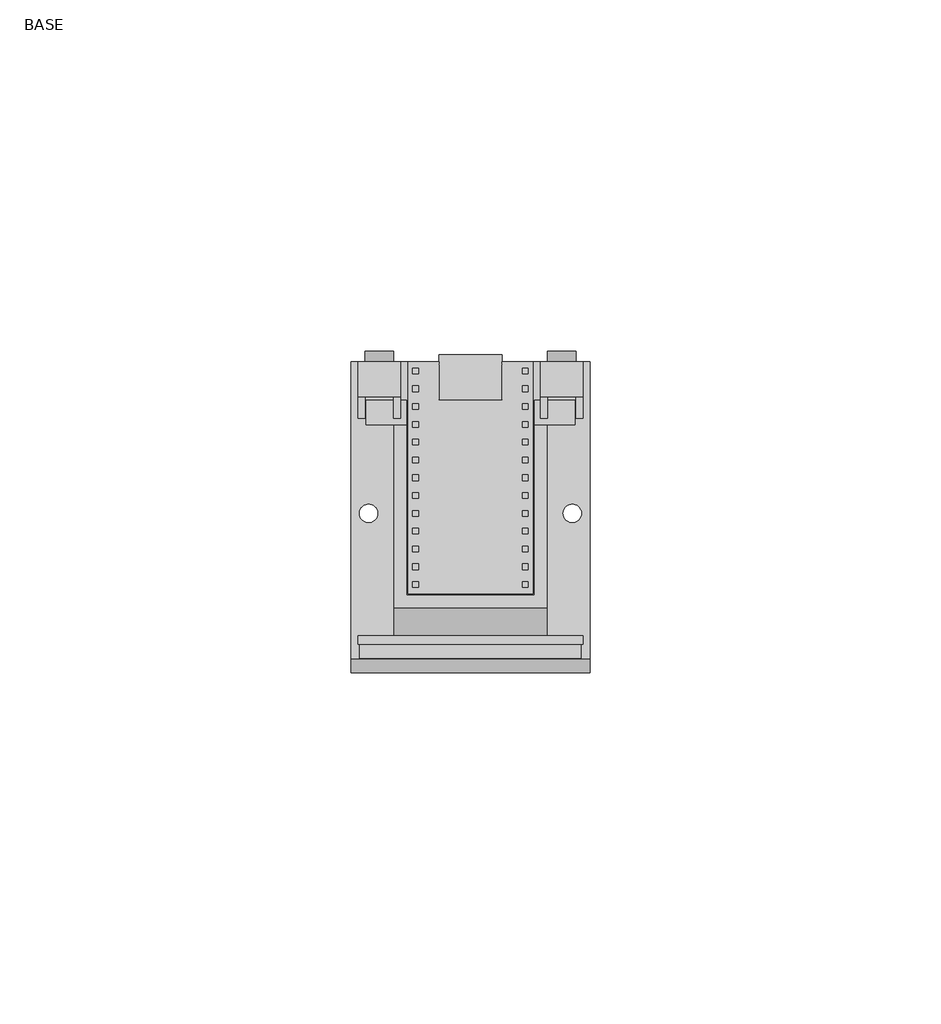
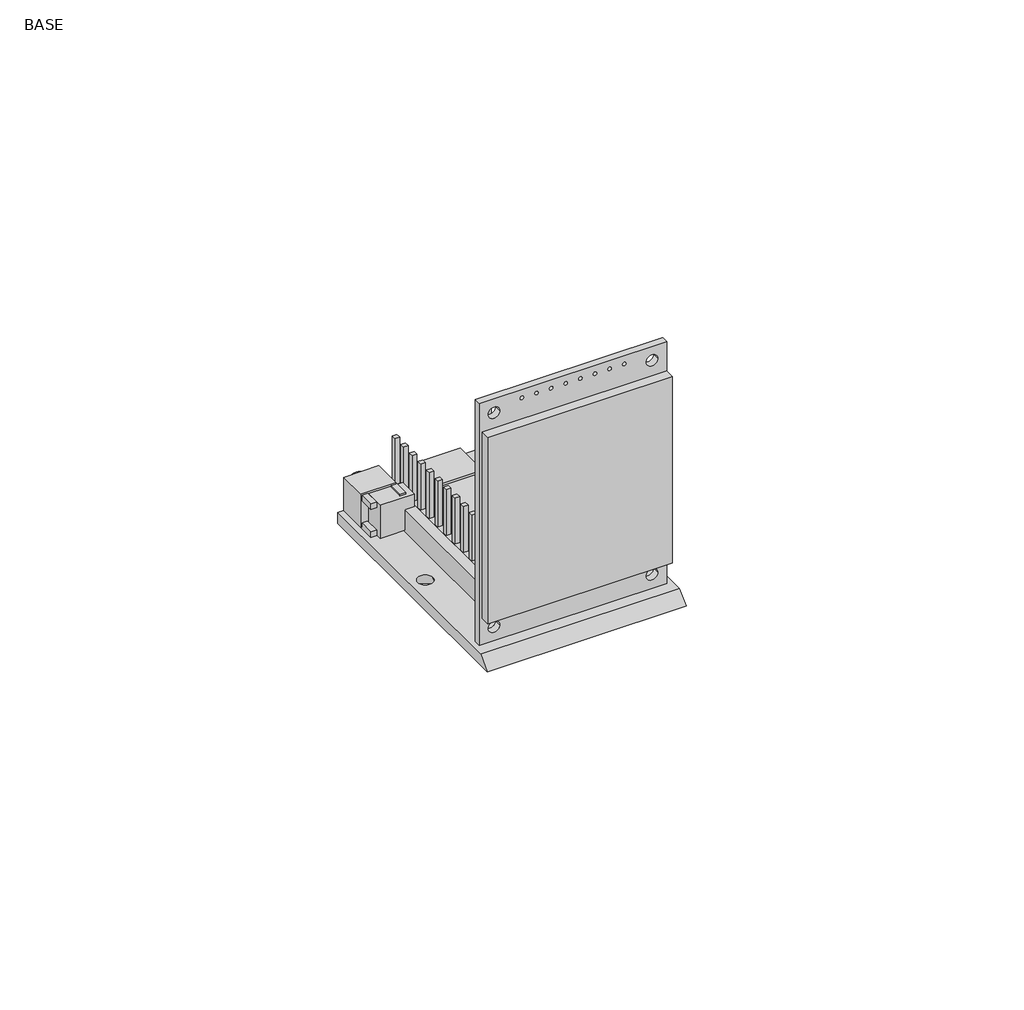
# One storey: 4 furniture elements, 1 proxy.
"""IFC4 building model written with IfcOpenShell, lengths in millimetres."""

import ifcopenshell
import ifcopenshell.guid

model = None  # the IFC model being written
_history = None  # IfcOwnerHistory: only IFC2X3 demands one
_inside = {}  # id of a spatial element -> (the spatial element, [elements in it])
_under = {}  # id of a project, library or spatial element -> (it, [spatial elements below it])
_declared = {}  # id of a project -> (the project, [libraries it declares])
_typed = {}  # id of a type object -> (the type object, [elements of that type])
_made_of = {}  # id of a material, layer set ... -> (it, [elements and type objects made of it])


def new_model(schema):
    """Start an empty IFC model of exactly this schema.

    Asked for "IFC4X3", IfcOpenShell would pick the latest addendum, in which some entities
    have other attributes; the version numbers below select the first issue.
    IFC2X3 requires an IfcOwnerHistory on every rooted entity: one is made here for all.
    """
    global model, _history
    if schema == "IFC4X3":
        model = ifcopenshell.file(schema_version=(4, 3, 0, 0))
    else:
        model = ifcopenshell.file(schema=schema)
    _inside.clear()
    _under.clear()
    _declared.clear()
    _typed.clear()
    _made_of.clear()
    _history = None
    if model.schema == "IFC2X3":
        org = make("IfcOrganization", Name="unknown")
        user = make(
            "IfcPersonAndOrganization",
            ThePerson=make("IfcPerson", FamilyName="unknown"),
            TheOrganization=org,
        )
        app = make(
            "IfcApplication",
            ApplicationDeveloper=org,
            Version="unknown",
            ApplicationFullName="unknown",
            ApplicationIdentifier="unknown",
        )
        _history = make(
            "IfcOwnerHistory",
            OwningUser=user,
            OwningApplication=app,
            ChangeAction="ADDED",
            CreationDate=0,
        )
    return model


def make(cls, **values):
    """One entity of the class cls with the attributes given. An attribute that is None is left unset."""
    return model.create_entity(
        cls, **{name: value for name, value in values.items() if value is not None}
    )


def rooted(cls, **values):
    """An entity with a GlobalId (a new one), such as an element, a storey or a relation."""
    return make(cls, GlobalId=ifcopenshell.guid.new(), OwnerHistory=_history, **values)


def si_unit(unit_type, name, prefix=None):
    """IfcSIUnit, for example si_unit("LENGTHUNIT", "METRE", prefix="MILLI")."""
    return make("IfcSIUnit", UnitType=unit_type, Prefix=prefix, Name=name)


def assignment(units):
    """IfcUnitAssignment: the units of a project."""
    return None if units is None else make("IfcUnitAssignment", Units=units)


def point(xyz):
    """IfcCartesianPoint."""
    return None if xyz is None else make("IfcCartesianPoint", Coordinates=xyz)


def direction(xyz):
    """IfcDirection."""
    return None if xyz is None else make("IfcDirection", DirectionRatios=xyz)


def frame(location, z_axis=None, x_axis=None):
    """IfcAxis2Placement3D, a coordinate frame: its origin and axes. An axis left out is left unset."""
    return make(
        "IfcAxis2Placement3D",
        Location=point(location),
        Axis=direction(z_axis),
        RefDirection=direction(x_axis),
    )


def frame_2d(location, x_axis=None):
    """IfcAxis2Placement2D, a coordinate frame in the plane: its origin and x axis."""
    return make(
        "IfcAxis2Placement2D", Location=point(location), RefDirection=direction(x_axis)
    )


def origin():
    """The frame at (0, 0, 0) with its axes left unset."""
    return frame((0.0, 0.0, 0.0))


def origin_with_axes():
    """The frame at (0, 0, 0) with the z axis (0, 0, 1) and the x axis (1, 0, 0) written out."""
    return frame((0.0, 0.0, 0.0), z_axis=(0.0, 0.0, 1.0), x_axis=(1.0, 0.0, 0.0))


def place(relative_to, where):
    """IfcLocalPlacement: puts the frame where relative to a parent placement (None: the world)."""
    return make(
        "IfcLocalPlacement", PlacementRelTo=relative_to, RelativePlacement=where
    )


def context(
    kind, dimensions, precision=None, world=None, true_north=None, identifier=None
):
    """IfcGeometricRepresentationContext, for example the 3D "Model" context."""
    return make(
        "IfcGeometricRepresentationContext",
        ContextIdentifier=identifier,
        ContextType=kind,
        CoordinateSpaceDimension=dimensions,
        Precision=precision,
        WorldCoordinateSystem=world,
        TrueNorth=true_north,
    )


def project(units=None, contexts=None):
    """IfcProject with its units and contexts."""
    return rooted(
        "IfcProject",
        Name="project",
        RepresentationContexts=contexts,
        UnitsInContext=assignment(units),
    )


def spatial(cls, under=None, at=None, **own):
    """A site, building, storey or space (cls), placed at a placement, below another one or the project."""
    s = rooted(cls, ObjectPlacement=at, **own)
    if under is not None:
        _under.setdefault(under.id(), (under, []))[1].append(s)
    return s


def polyline(points):
    """IfcPolyline through the points."""
    return make("IfcPolyline", Points=[point(p) for p in points])


def circle_curve(where, radius):
    """IfcCircle in the frame where."""
    return make("IfcCircle", Position=where, Radius=radius)


def trimmed(basis, trim1, trim2, sense, master):
    """IfcTrimmedCurve: the piece of a basis curve between two trims."""
    return make(
        "IfcTrimmedCurve",
        BasisCurve=basis,
        Trim1=trim1,
        Trim2=trim2,
        SenseAgreement=sense,
        MasterRepresentation=master,
    )


def segment(curve, same_sense, transition):
    """IfcCompositeCurveSegment."""
    return make(
        "IfcCompositeCurveSegment",
        Transition=transition,
        SameSense=same_sense,
        ParentCurve=curve,
    )


def composite_curve(segments, self_intersect=None):
    """IfcCompositeCurve: segments joined end to end."""
    return make("IfcCompositeCurve", Segments=segments, SelfIntersect=self_intersect)


def outline(outer, holes=None, kind="AREA"):
    """IfcArbitraryClosedProfileDef: a profile drawn as a closed curve; with holes, ...WithVoids."""
    if holes is None:
        return make("IfcArbitraryClosedProfileDef", ProfileType=kind, OuterCurve=outer)
    return make(
        "IfcArbitraryProfileDefWithVoids",
        ProfileType=kind,
        OuterCurve=outer,
        InnerCurves=holes,
    )


def extrude(swept, where, along, depth):
    """IfcExtrudedAreaSolid: the profile swept, set in the frame where, extruded along a direction by depth."""
    return make(
        "IfcExtrudedAreaSolid",
        SweptArea=swept,
        Position=where,
        ExtrudedDirection=direction(along),
        Depth=depth,
    )


def faces_of(points, faces, orient=None, outer=None):
    """IfcFace entities. A face is a list of loops; a loop is a list of indices into points, from 0.

    orient and outer hold one flag for each loop. By default every Orientation is true, the
    first loop of a face is its IfcFaceOuterBound and the others are IfcFaceBound.
    """
    made = []
    for i, loops in enumerate(faces):
        bounds = []
        for j, loop in enumerate(loops):
            is_outer = j == 0 if outer is None else outer[i][j]
            bounds.append(
                make(
                    "IfcFaceOuterBound" if is_outer else "IfcFaceBound",
                    Bound=make("IfcPolyLoop", Polygon=[points[k] for k in loop]),
                    Orientation=True if orient is None else orient[i][j],
                )
            )
        made.append(make("IfcFace", Bounds=bounds))
    return made


def faceted_brep(points, faces, orient=None, outer=None, voids=None):
    """IfcFacetedBrep: a solid bounded by flat faces; with voids (closed shells), ...WithVoids."""
    shared = [point(p) for p in points]
    hull = make("IfcClosedShell", CfsFaces=faces_of(shared, faces, orient, outer))
    if voids is None:
        return make("IfcFacetedBrep", Outer=hull)
    return make(
        "IfcFacetedBrepWithVoids",
        Outer=hull,
        Voids=[
            make(cls, CfsFaces=faces_of(shared, fs, o, b)) for cls, fs, o, b in voids
        ],
    )


def shape(context_of_items, identifier, shape_type, items):
    """IfcShapeRepresentation: the items that make up one representation, for example the "Body"."""
    return make(
        "IfcShapeRepresentation",
        ContextOfItems=context_of_items,
        RepresentationIdentifier=identifier,
        RepresentationType=shape_type,
        Items=items,
    )


def source(mapping_origin, context_of_items, identifier, shape_type, items):
    """IfcRepresentationMap: a shape defined once, which mapped items show again and again."""
    return make(
        "IfcRepresentationMap",
        MappingOrigin=mapping_origin,
        MappedRepresentation=shape(context_of_items, identifier, shape_type, items),
    )


def transform(
    local_origin,
    x_axis=None,
    y_axis=None,
    z_axis=None,
    scale=None,
    scale2=None,
    scale3=None,
    uniform=True,
):
    """IfcCartesianTransformationOperator3D, or its non-uniform kind. x_axis, y_axis, z_axis: its Axis1, 2, 3."""
    if uniform:
        return make(
            "IfcCartesianTransformationOperator3D",
            Axis1=direction(x_axis),
            Axis2=direction(y_axis),
            LocalOrigin=point(local_origin),
            Scale=scale,
            Axis3=direction(z_axis),
        )
    return make(
        "IfcCartesianTransformationOperator3DnonUniform",
        Axis1=direction(x_axis),
        Axis2=direction(y_axis),
        LocalOrigin=point(local_origin),
        Scale=scale,
        Axis3=direction(z_axis),
        Scale2=scale2,
        Scale3=scale3,
    )


def mapped(mapping_source, mapping_target):
    """IfcMappedItem: shows the shape of a source again, moved by a transform."""
    return make(
        "IfcMappedItem", MappingSource=mapping_source, MappingTarget=mapping_target
    )


def made_of(thing, what):
    """Note that an element or type object is made of a material, layer set ...; save() writes the relation."""
    if what is not None:
        _made_of.setdefault(what.id(), (what, []))[1].append(thing)
    return thing


def element(
    cls,
    number,
    at=None,
    inside=None,
    cuts=None,
    type_object=None,
    material=None,
    context=None,
    identifier="Body",
    shape_type=None,
    held_by="IfcProductDefinitionShape",
    body=None,
    shapes=None,
    **own,
):
    """One element of the class cls, such as IfcWall. Its Tag is "e" and its number.

    at: its placement. inside: the storey or other place that contains it. cuts: it is an
    opening in that element (IfcRelVoidsElement). A single representation is given by context,
    identifier, shape_type and body (its items); several are given by shapes. held_by: the class
    of the entity that holds the representations. save() writes the other relations.
    """
    e = rooted(cls, Tag="e%d" % number, ObjectPlacement=at, **own)
    if body is not None:
        shapes = [shape(context, identifier, shape_type, body)]
    if shapes is not None:
        e.Representation = make(held_by, Representations=shapes)
    if inside is not None:
        _inside.setdefault(inside.id(), (inside, []))[1].append(e)
    if cuts is not None:
        rooted(
            "IfcRelVoidsElement", RelatingBuildingElement=cuts, RelatedOpeningElement=e
        )
    if type_object is not None:
        _typed.setdefault(type_object.id(), (type_object, []))[1].append(e)
    return made_of(e, material)


def aggregate(whole, parts):
    """IfcRelAggregates: a whole, such as a stair, and the parts it consists of."""
    return rooted("IfcRelAggregates", RelatingObject=whole, RelatedObjects=parts)


def save(model, path):
    """Write the relations noted so far, then the file.

    IfcRelAggregates (storeys below a building ...), IfcRelContainedInSpatialStructure (elements
    in a storey), IfcRelDefinesByType, IfcRelAssociatesMaterial and IfcRelDeclares: one each for
    every whole, place, type object, material and project.
    """
    for whole, parts in _under.values():
        aggregate(whole, parts)
    for where, things in _inside.values():
        rooted(
            "IfcRelContainedInSpatialStructure",
            RelatedElements=things,
            RelatingStructure=where,
        )
    for kind, things in _typed.values():
        rooted("IfcRelDefinesByType", RelatedObjects=things, RelatingType=kind)
    for what, things in _made_of.values():
        rooted("IfcRelAssociatesMaterial", RelatedObjects=things, RelatingMaterial=what)
    for by, libraries in _declared.values():
        rooted("IfcRelDeclares", RelatingContext=by, RelatedDefinitions=libraries)
    model.write(path)


def plane_surface(at):
    """IfcPlane: the flat surface through the origin of the frame at, square to its z axis."""
    return make("IfcPlane", Position=at)


def revolved_surface(curve, axis_point, axis_direction):
    """IfcSurfaceOfRevolution: the curve turned about the line through axis_point along axis_direction."""
    return make(
        "IfcSurfaceOfRevolution",
        SweptCurve=make("IfcArbitraryOpenProfileDef", ProfileType="CURVE", Curve=curve),
        AxisPosition=make("IfcAxis1Placement", Location=point(axis_point), Axis=direction(axis_direction)),
    )


def advanced_brep(points, edges, surfaces, faces):
    """IfcAdvancedBrep: a solid bounded by faces that lie on surfaces and meet in shared edges.

    An edge is (start, end): straight between two places in points (the first is 0);
    or (start, end, curve); or (start, end, curve, False) where it runs against its curve.
    A face is (place in surfaces, loops), or (place, loops, False) where it looks against
    its surface's normal. A loop lists edges by number (the first is 1), with a minus sign
    where the edge is run from its end to its start. The first loop is the outer one.
    """
    corners = [point(p) for p in points]
    vertices = [make("IfcVertexPoint", VertexGeometry=c) for c in corners]
    made = []
    for start, end, *more in edges:
        made.append(
            make(
                "IfcEdgeCurve",
                EdgeStart=vertices[start],
                EdgeEnd=vertices[end],
                EdgeGeometry=more[0] if more else make("IfcPolyline", Points=[corners[start], corners[end]]),
                SameSense=more[1] if len(more) > 1 else True,
            )
        )
    hull = []
    for where, loops, *sense in faces:
        bounds = []
        for j, loop in enumerate(loops):
            ring = [make("IfcOrientedEdge", EdgeElement=made[abs(k) - 1], Orientation=k > 0) for k in loop]
            bounds.append(
                make(
                    "IfcFaceOuterBound" if j == 0 else "IfcFaceBound",
                    Bound=make("IfcEdgeLoop", EdgeList=ring),
                    Orientation=True,
                )
            )
        hull.append(make("IfcAdvancedFace", Bounds=bounds, FaceSurface=surfaces[where], SameSense=sense[0] if sense else True))
    return make("IfcAdvancedBrep", Outer=make("IfcClosedShell", CfsFaces=hull))


def case_case_ec59ddf9(model_context):
    return source(origin(), model_context, "Body", "SolidModel", [
        extrude(outline(polyline([(1461.1150176, 13229.1739696), (1466.9150176, 13229.1739696), (1466.9150176, 13225.7186096), (1461.1150176, 13225.7186096), (1461.1150176, 13229.1739696)])), frame((0.0, 0.0, 2.0), z_axis=(0.0, 0.0, 1.0), x_axis=(1.0, 0.0, 0.0)), (0.0, 0.0, 1.0), 6.0),
        extrude(outline(polyline([(1442.9350176, 13229.1739696), (1442.9350176, 13225.7186096), (1437.1350176, 13225.7186096), (1437.1350176, 13229.1739696), (1442.9350176, 13229.1739696)])), frame((0.0, 0.0, 2.0), z_axis=(0.0, 0.0, 1.0), x_axis=(1.0, 0.0, 0.0)), (0.0, 0.0, 1.0), 6.0),
        advanced_brep(
        [(1469.0250176, 13192.4212784, 2.0), (1469.0250176, 13234.6739696, 2.0), (1435.0250176, 13234.6739696, 2.0), (1435.0250176, 13192.4212784, 2.0), (1441.1350176, 13195.6739696, 2.0), (1441.1350176, 13225.7186096, 2.0), (1442.9350176, 13225.7186096, 2.0), (1442.9350176, 13201.4739696, 2.0), (1461.1150176, 13201.4739696, 2.0), (1461.1150176, 13225.7186096, 2.0), (1462.9150176, 13225.7186096, 2.0), (1462.9150176, 13195.6739696, 2.0), (1467.8250176, 13213.1041412, 2.0), (1465.2250176, 13213.1041412, 2.0), (1438.8250176, 13213.1041412, 2.0), (1436.2250176, 13213.1041412, 2.0), (1435.0250176, 13234.6739696, 0.0), (1469.0250176, 13234.6739696, 0.0), (1469.0250176, 13190.4212784, 0.0), (1435.0250176, 13190.4212784, 0.0), (1464.5250176, 13213.1041412, 0.0), (1468.5250176, 13213.1041412, 0.0), (1435.5250176, 13213.1041412, 0.0), (1439.5250176, 13213.1041412, 0.0), (1441.1350176, 13225.7186096, 6.0), (1441.1350176, 13199.6739696, 6.0), (1462.9150176, 13199.6739696, 6.0), (1462.9150176, 13225.7186096, 6.0), (1461.1150176, 13225.7186096, 6.0), (1461.1150176, 13201.4739696, 6.0), (1442.9350176, 13201.4739696, 6.0), (1442.9350176, 13225.7186096, 6.0)],
        [
            (0, 1),
            (1, 2),
            (2, 3),
            (3, 0),
            (4, 5),
            (5, 6),
            (6, 7),
            (7, 8),
            (8, 9),
            (9, 10),
            (10, 11),
            (11, 4),
            (12, 13, circle_curve(frame((1466.5250176, 13213.1041412, 2.0), z_axis=(0.0, 0.0, -1.0), x_axis=(-1.0, 0.0, 0.0)), 1.3)),
            (13, 12, circle_curve(frame((1466.5250176, 13213.1041412, 2.0), z_axis=(0.0, 0.0, -1.0), x_axis=(1.0, 0.0, 0.0)), 1.3)),
            (14, 15, circle_curve(frame((1437.5250176, 13213.1041412, 2.0), z_axis=(0.0, 0.0, -1.0), x_axis=(-1.0, 0.0, 0.0)), 1.3)),
            (15, 14, circle_curve(frame((1437.5250176, 13213.1041412, 2.0), z_axis=(0.0, 0.0, -1.0), x_axis=(1.0, 0.0, 0.0)), 1.3)),
            (16, 17),
            (17, 18),
            (18, 19),
            (19, 16),
            (20, 21, circle_curve(frame((1466.5250176, 13213.1041412, 0.0), z_axis=(0.0, 0.0, 1.0), x_axis=(-1.0, 0.0, 0.0)), 2.0)),
            (21, 20, circle_curve(frame((1466.5250176, 13213.1041412, 0.0), z_axis=(0.0, 0.0, 1.0), x_axis=(1.0, 0.0, 0.0)), 2.0)),
            (22, 23, circle_curve(frame((1437.5250176, 13213.1041412, 0.0), z_axis=(0.0, 0.0, 1.0), x_axis=(-1.0, 0.0, 0.0)), 2.0)),
            (23, 22, circle_curve(frame((1437.5250176, 13213.1041412, 0.0), z_axis=(0.0, 0.0, 1.0), x_axis=(1.0, 0.0, 0.0)), 2.0)),
            (0, 18),
            (17, 1),
            (16, 2),
            (19, 3),
            (24, 25),
            (25, 26),
            (26, 27),
            (27, 28),
            (28, 29),
            (29, 30),
            (30, 31),
            (31, 24),
            (24, 5),
            (4, 25),
            (26, 11),
            (10, 27),
            (9, 28),
            (8, 29),
            (7, 30),
            (6, 31),
            (20, 13),
            (12, 21),
            (22, 15),
            (14, 23),
        ],
        [
            plane_surface(frame((1467.7850176, 13192.4212784, 2.0), z_axis=(0.0, 0.0, 1.0), x_axis=(1.0, 0.0, 0.0))),
            plane_surface(frame((1467.7850176, 13192.4212784, 0.0), z_axis=(0.0, 0.0, -1.0), x_axis=(-1.0, 0.0, 0.0))),
            plane_surface(frame((1469.0250176, 13192.4212784, 2.0), z_axis=(1.0, 0.0, 0.0), x_axis=(0.0, 0.0, -1.0))),
            plane_surface(frame((1469.0250176, 13234.6739696, 2.0), z_axis=(0.0, 1.0, 0.0), x_axis=(0.0, 0.0, -1.0))),
            plane_surface(frame((1435.0250176, 13234.6739696, 2.0), z_axis=(-1.0, 0.0, 0.0), x_axis=(0.0, 0.0, -1.0))),
            plane_surface(frame((1441.1350176, 13234.6739696, 6.0), z_axis=(0.0, 0.0, 1.0), x_axis=(0.0, -1.0, 0.0))),
            plane_surface(frame((1441.1350176, 13225.7186096, 6.0), z_axis=(-1.0, 0.0, 0.0), x_axis=(0.0, 0.0, -1.0))),
            plane_surface(frame((1462.9150176, 13199.6739696, 6.0), z_axis=(1.0, 0.0, 0.0), x_axis=(0.0, 0.0, -1.0))),
            plane_surface(frame((1462.9150176, 13225.7186096, 6.0), z_axis=(0.0, 1.0, 0.0), x_axis=(0.0, 0.0, -1.0))),
            plane_surface(frame((1461.1150176, 13225.7186096, 6.0), z_axis=(-1.0, 0.0, 0.0), x_axis=(0.0, 0.0, -1.0))),
            plane_surface(frame((1461.1150176, 13201.4739696, 6.0), z_axis=(0.0, 1.0, 0.0), x_axis=(0.0, 0.0, -1.0))),
            plane_surface(frame((1442.9350176, 13201.4739696, 6.0), z_axis=(1.0, 0.0, 0.0), x_axis=(0.0, 0.0, -1.0))),
            plane_surface(frame((1442.9350176, 13225.7186096, 6.0), z_axis=(0.0, 1.0, 0.0), x_axis=(0.0, 0.0, -1.0))),
            plane_surface(frame((1441.1350176, 13195.6739696, 2.0), z_axis=(0.0, -0.7071067811865885, 0.7071067811865066), x_axis=(1.0, 0.0, 0.0))),
            plane_surface(frame((1435.0250176, 13190.4212784, 0.0), z_axis=(0.0, -0.707106781186628, 0.7071067811864672), x_axis=(1.0, 0.0, 0.0))),
            revolved_surface(polyline([(1464.5250176, 13213.1041412, 0.0), (1465.2250176017499, 13213.1041412, 2.0)]), (1466.5250176, 13213.1041412, 5.7142857), (0.0, 0.0, -1.0)),
            revolved_surface(polyline([(1435.5250176, 13213.1041412, 0.0), (1436.2250176017499, 13213.1041412, 2.0)]), (1437.5250176, 13213.1041412, 5.7142857), (0.0, 0.0, -1.0)),
        ],
        [
            (0, [[1, 2, 3, 4], [5, 6, 7, 8, 9, 10, 11, 12], [13, 14], [15, 16]]),
            (1, [[17, 18, 19, 20], [21, 22], [23, 24]]),
            (2, [[-1, 25, -18, 26]]),
            (3, [[-2, -26, -17, 27]]),
            (4, [[-3, -27, -20, 28]]),
            (5, [[29, 30, 31, 32, 33, 34, 35, 36]]),
            (6, [[-29, 37, -5, 38]]),
            (7, [[-31, 39, -11, 40]]),
            (8, [[-32, -40, -10, 41]]),
            (9, [[-33, -41, -9, 42]]),
            (10, [[-34, -42, -8, 43]]),
            (11, [[-35, -43, -7, 44]]),
            (12, [[-36, -44, -6, -37]]),
            (13, [[-38, -12, -39, -30]]),
            (14, [[-28, -19, -25, -4]]),
            (15, [[45, -13, 46, -21]]),
            (15, [[-45, -22, -46, -14]]),
            (16, [[47, -15, 48, -23]]),
            (16, [[-47, -24, -48, -16]]),
        ],
    ),
    ])


def furniture_1_54tft_screen_1_54tft_screen_d9e98271(model_context):
    return source(origin(), model_context, "Body", "SweptSolid", [
        extrude(outline(polyline([(43.7, 16.0), (43.7, -16.0), (0.0, -16.0), (0.0, 16.0), (43.7, 16.0)]), holes=[composite_curve([segment(trimmed(circle_curve(frame_2d((2.5, 13.5)), 1.0), [point((2.5, 14.5))], [point((2.5, 12.5))], True, "CARTESIAN"), True, "CONTINUOUS"), segment(trimmed(circle_curve(frame_2d((2.5, 13.5)), 1.0), [point((2.5, 12.5))], [point((2.5, 14.5))], True, "CARTESIAN"), True, "CONTINUOUS")], self_intersect=False), composite_curve([segment(trimmed(circle_curve(frame_2d((41.2, 13.5)), 1.0), [point((41.2, 14.5))], [point((41.2, 12.5))], True, "CARTESIAN"), True, "CONTINUOUS"), segment(trimmed(circle_curve(frame_2d((41.2, 13.5)), 1.0), [point((41.2, 12.5))], [point((41.2, 14.5))], True, "CARTESIAN"), True, "CONTINUOUS")], self_intersect=False), composite_curve([segment(trimmed(circle_curve(frame_2d((42.2, -1.25)), 0.3), [point((42.2, -0.95))], [point((42.2, -1.55))], True, "CARTESIAN"), True, "CONTINUOUS"), segment(trimmed(circle_curve(frame_2d((42.2, -1.25)), 0.3), [point((42.2, -1.55))], [point((42.2, -0.95))], True, "CARTESIAN"), True, "CONTINUOUS")], self_intersect=False), composite_curve([segment(trimmed(circle_curve(frame_2d((42.2, 1.25)), 0.3), [point((42.2, 1.55))], [point((42.2, 0.95))], True, "CARTESIAN"), True, "CONTINUOUS"), segment(trimmed(circle_curve(frame_2d((42.2, 1.25)), 0.3), [point((42.2, 0.95))], [point((42.2, 1.55))], True, "CARTESIAN"), True, "CONTINUOUS")], self_intersect=False), composite_curve([segment(trimmed(circle_curve(frame_2d((42.2, 3.75)), 0.3), [point((42.2, 4.05))], [point((42.2, 3.45))], True, "CARTESIAN"), True, "CONTINUOUS"), segment(trimmed(circle_curve(frame_2d((42.2, 3.75)), 0.3), [point((42.2, 3.45))], [point((42.2, 4.05))], True, "CARTESIAN"), True, "CONTINUOUS")], self_intersect=False), composite_curve([segment(trimmed(circle_curve(frame_2d((42.2, 6.25)), 0.3), [point((42.2, 6.55))], [point((42.2, 5.95))], True, "CARTESIAN"), True, "CONTINUOUS"), segment(trimmed(circle_curve(frame_2d((42.2, 6.25)), 0.3), [point((42.2, 5.95))], [point((42.2, 6.55))], True, "CARTESIAN"), True, "CONTINUOUS")], self_intersect=False), composite_curve([segment(trimmed(circle_curve(frame_2d((42.2, 8.75)), 0.3), [point((42.2, 9.05))], [point((42.2, 8.45))], True, "CARTESIAN"), True, "CONTINUOUS"), segment(trimmed(circle_curve(frame_2d((42.2, 8.75)), 0.3), [point((42.2, 8.45))], [point((42.2, 9.05))], True, "CARTESIAN"), True, "CONTINUOUS")], self_intersect=False), composite_curve([segment(trimmed(circle_curve(frame_2d((42.2, -3.75)), 0.3), [point((42.2, -3.45))], [point((42.2, -4.05))], True, "CARTESIAN"), True, "CONTINUOUS"), segment(trimmed(circle_curve(frame_2d((42.2, -3.75)), 0.3), [point((42.2, -4.05))], [point((42.2, -3.45))], True, "CARTESIAN"), True, "CONTINUOUS")], self_intersect=False), composite_curve([segment(trimmed(circle_curve(frame_2d((42.2, -6.25)), 0.3), [point((42.2, -5.95))], [point((42.2, -6.55))], True, "CARTESIAN"), True, "CONTINUOUS"), segment(trimmed(circle_curve(frame_2d((42.2, -6.25)), 0.3), [point((42.2, -6.55))], [point((42.2, -5.95))], True, "CARTESIAN"), True, "CONTINUOUS")], self_intersect=False), composite_curve([segment(trimmed(circle_curve(frame_2d((42.2, -8.75)), 0.3), [point((42.2, -8.45))], [point((42.2, -9.05))], True, "CARTESIAN"), True, "CONTINUOUS"), segment(trimmed(circle_curve(frame_2d((42.2, -8.75)), 0.3), [point((42.2, -9.05))], [point((42.2, -8.45))], True, "CARTESIAN"), True, "CONTINUOUS")], self_intersect=False), composite_curve([segment(trimmed(circle_curve(frame_2d((41.2, -13.5)), 1.0), [point((41.2, -14.5))], [point((41.2, -12.5))], True, "CARTESIAN"), True, "CONTINUOUS"), segment(trimmed(circle_curve(frame_2d((41.2, -13.5)), 1.0), [point((41.2, -12.5))], [point((41.2, -14.5))], True, "CARTESIAN"), True, "CONTINUOUS")], self_intersect=False), composite_curve([segment(trimmed(circle_curve(frame_2d((2.5, -13.5)), 1.0), [point((2.5, -14.5))], [point((2.5, -12.5))], True, "CARTESIAN"), True, "CONTINUOUS"), segment(trimmed(circle_curve(frame_2d((2.5, -13.5)), 1.0), [point((2.5, -12.5))], [point((2.5, -14.5))], True, "CARTESIAN"), True, "CONTINUOUS")], self_intersect=False)]), frame((0.0, -1.2, 0.0), z_axis=(0.0, 1.0, 0.0), x_axis=(0.0, 0.0, 1.0)), (0.0, 0.0, 1.0), 1.2),
        extrude(outline(polyline([(15.76, -1.3), (15.76, -3.2), (-15.76, -3.2), (-15.76, -1.3), (15.76, -1.3)])), frame((0.0, 0.0, 5.0), z_axis=(0.0, 0.0, 1.0), x_axis=(1.0, 0.0, 0.0)), (0.0, 0.0, 1.0), 33.7),
        extrude(outline(polyline([(13.86, -2.3592442), (13.86, -3.2), (-13.86, -3.2), (-13.86, -2.3592442), (13.86, -2.3592442)])), frame((0.0, 0.0, 9.5994076), z_axis=(0.0, 0.0, 1.0), x_axis=(1.0, 0.0, 0.0)), (0.0, 0.0, 1.0), 27.7),
    ])


def pro_micro_nrf52840_pro_micro_nrf52840_bcfd0b97(model_context):
    return source(origin(), model_context, "Body", "Brep", [
        faceted_brep([(-14.8, 8.2144911, 11.3), (-15.6, 8.2144911, 11.3), (-15.6, 7.4144911, 11.3), (-14.8, 7.4144911, 11.3), (15.6, 8.2144911, 11.3), (14.8, 8.2144911, 11.3), (14.8, 7.4144911, 11.3), (15.6, 7.4144911, 11.3), (13.0666667, 8.2144911, 11.3), (12.2666667, 8.2144911, 11.3), (12.2666667, 7.4144911, 11.3), (13.0666667, 7.4144911, 11.3), (10.5333333, 8.2144911, 11.3), (9.7333333, 8.2144911, 11.3), (9.7333333, 7.4144911, 11.3), (10.5333333, 7.4144911, 11.3), (8.0, 8.2144911, 11.3), (7.2, 8.2144911, 11.3), (7.2, 7.4144911, 11.3), (8.0, 7.4144911, 11.3), (5.4666667, 8.2144911, 11.3), (4.6666667, 8.2144911, 11.3), (4.6666667, 7.4144911, 11.3), (5.4666667, 7.4144911, 11.3), (2.9333333, 8.2144911, 11.3), (2.1333333, 8.2144911, 11.3), (2.1333333, 7.4144911, 11.3), (2.9333333, 7.4144911, 11.3), (0.4, 8.2144911, 11.3), (-0.4, 8.2144911, 11.3), (-0.4, 7.4144911, 11.3), (0.4, 7.4144911, 11.3), (-2.1333333, 8.2144911, 11.3), (-2.9333333, 8.2144911, 11.3), (-2.9333333, 7.4144911, 11.3), (-2.1333333, 7.4144911, 11.3), (-4.6666667, 8.2144911, 11.3), (-5.4666667, 8.2144911, 11.3), (-5.4666667, 7.4144911, 11.3), (-4.6666667, 7.4144911, 11.3), (-7.2, 8.2144911, 11.3), (-8.0, 8.2144911, 11.3), (-8.0, 7.4144911, 11.3), (-7.2, 7.4144911, 11.3), (-9.7333333, 8.2144911, 11.3), (-10.5333333, 8.2144911, 11.3), (-10.5333333, 7.4144911, 11.3), (-9.7333333, 7.4144911, 11.3), (-12.2666667, 8.2144911, 11.3), (-13.0666667, 8.2144911, 11.3), (-13.0666667, 7.4144911, 11.3), (-12.2666667, 7.4144911, 11.3), (-14.8, 8.2144911, 0.0), (-14.8, 7.4144911, 0.0), (-15.6, 7.4144911, 0.0), (-15.6, 8.2144911, 0.0), (15.6, 8.2144911, 0.0), (15.6, 7.4144911, 0.0), (14.8, 7.4144911, 0.0), (14.8, 8.2144911, 0.0), (13.0666667, 8.2144911, 0.0), (13.0666667, 7.4144911, 0.0), (12.2666667, 7.4144911, 0.0), (12.2666667, 8.2144911, 0.0), (10.5333333, 8.2144911, 0.0), (10.5333333, 7.4144911, 0.0), (9.7333333, 7.4144911, 0.0), (9.7333333, 8.2144911, 0.0), (8.0, 8.2144911, 0.0), (8.0, 7.4144911, 0.0), (7.2, 7.4144911, 0.0), (7.2, 8.2144911, 0.0), (5.4666667, 8.2144911, 0.0), (5.4666667, 7.4144911, 0.0), (4.6666667, 7.4144911, 0.0), (4.6666667, 8.2144911, 0.0), (2.9333333, 8.2144911, 0.0), (2.9333333, 7.4144911, 0.0), (2.1333333, 7.4144911, 0.0), (2.1333333, 8.2144911, 0.0), (0.4, 8.2144911, 0.0), (0.4, 7.4144911, 0.0), (-0.4, 7.4144911, 0.0), (-0.4, 8.2144911, 0.0), (-2.1333333, 8.2144911, 0.0), (-2.1333333, 7.4144911, 0.0), (-2.9333333, 7.4144911, 0.0), (-2.9333333, 8.2144911, 0.0), (-4.6666667, 8.2144911, 0.0), (-4.6666667, 7.4144911, 0.0), (-5.4666667, 7.4144911, 0.0), (-5.4666667, 8.2144911, 0.0), (-7.2, 8.2144911, 0.0), (-7.2, 7.4144911, 0.0), (-8.0, 7.4144911, 0.0), (-8.0, 8.2144911, 0.0), (-9.7333333, 8.2144911, 0.0), (-9.7333333, 7.4144911, 0.0), (-10.5333333, 7.4144911, 0.0), (-10.5333333, 8.2144911, 0.0), (-12.2666667, 8.2144911, 0.0), (-12.2666667, 7.4144911, 0.0), (-13.0666667, 7.4144911, 0.0), (-13.0666667, 8.2144911, 0.0), (-14.8, 8.2144911, 3.0), (-15.6, 8.2144911, 3.0), (-15.6, 8.2144911, 1.0), (-14.8, 8.2144911, 1.0), (-15.6, 7.4144911, 3.0), (-15.6, 7.4144911, 1.0), (-14.8, 7.4144911, 3.0), (-14.8, 7.4144911, 1.0), (15.6, 8.2144911, 3.0), (14.8, 8.2144911, 3.0), (14.8, 8.2144911, 1.0), (15.6, 8.2144911, 1.0), (14.8, 7.4144911, 3.0), (14.8, 7.4144911, 1.0), (15.6, 7.4144911, 3.0), (15.6, 7.4144911, 1.0), (13.0666667, 8.2144911, 3.0), (12.2666667, 8.2144911, 3.0), (12.2666667, 8.2144911, 1.0), (13.0666667, 8.2144911, 1.0), (12.2666667, 7.4144911, 3.0), (12.2666667, 7.4144911, 1.0), (13.0666667, 7.4144911, 3.0), (13.0666667, 7.4144911, 1.0), (10.5333333, 8.2144911, 3.0), (9.7333333, 8.2144911, 3.0), (9.7333333, 8.2144911, 1.0), (10.5333333, 8.2144911, 1.0), (9.7333333, 7.4144911, 3.0), (9.7333333, 7.4144911, 1.0), (10.5333333, 7.4144911, 3.0), (10.5333333, 7.4144911, 1.0), (8.0, 8.2144911, 3.0), (7.2, 8.2144911, 3.0), (7.2, 8.2144911, 1.0), (8.0, 8.2144911, 1.0), (7.2, 7.4144911, 3.0), (7.2, 7.4144911, 1.0), (8.0, 7.4144911, 3.0), (8.0, 7.4144911, 1.0), (5.4666667, 8.2144911, 3.0), (4.6666667, 8.2144911, 3.0), (4.6666667, 8.2144911, 1.0), (5.4666667, 8.2144911, 1.0), (4.6666667, 7.4144911, 3.0), (4.6666667, 7.4144911, 1.0), (5.4666667, 7.4144911, 3.0), (5.4666667, 7.4144911, 1.0), (2.9333333, 8.2144911, 3.0), (2.1333333, 8.2144911, 3.0), (2.1333333, 8.2144911, 1.0), (2.9333333, 8.2144911, 1.0), (2.1333333, 7.4144911, 3.0), (2.1333333, 7.4144911, 1.0), (2.9333333, 7.4144911, 3.0), (2.9333333, 7.4144911, 1.0), (0.4, 8.2144911, 3.0), (-0.4, 8.2144911, 3.0), (-0.4, 8.2144911, 1.0), (0.4, 8.2144911, 1.0), (-0.4, 7.4144911, 3.0), (-0.4, 7.4144911, 1.0), (0.4, 7.4144911, 3.0), (0.4, 7.4144911, 1.0), (-2.1333333, 8.2144911, 3.0), (-2.9333333, 8.2144911, 3.0), (-2.9333333, 8.2144911, 1.0), (-2.1333333, 8.2144911, 1.0), (-2.9333333, 7.4144911, 3.0), (-2.9333333, 7.4144911, 1.0), (-2.1333333, 7.4144911, 3.0), (-2.1333333, 7.4144911, 1.0), (-4.6666667, 8.2144911, 3.0), (-5.4666667, 8.2144911, 3.0), (-5.4666667, 8.2144911, 1.0), (-4.6666667, 8.2144911, 1.0), (-5.4666667, 7.4144911, 3.0), (-5.4666667, 7.4144911, 1.0), (-4.6666667, 7.4144911, 3.0), (-4.6666667, 7.4144911, 1.0), (-7.2, 8.2144911, 3.0), (-8.0, 8.2144911, 3.0), (-8.0, 8.2144911, 1.0), (-7.2, 8.2144911, 1.0), (-8.0, 7.4144911, 3.0), (-8.0, 7.4144911, 1.0), (-7.2, 7.4144911, 3.0), (-7.2, 7.4144911, 1.0), (-9.7333333, 8.2144911, 3.0), (-10.5333333, 8.2144911, 3.0), (-10.5333333, 8.2144911, 1.0), (-9.7333333, 8.2144911, 1.0), (-10.5333333, 7.4144911, 3.0), (-10.5333333, 7.4144911, 1.0), (-9.7333333, 7.4144911, 3.0), (-9.7333333, 7.4144911, 1.0), (-12.2666667, 8.2144911, 3.0), (-13.0666667, 8.2144911, 3.0), (-13.0666667, 8.2144911, 1.0), (-12.2666667, 8.2144911, 1.0), (-13.0666667, 7.4144911, 3.0), (-13.0666667, 7.4144911, 1.0), (-12.2666667, 7.4144911, 3.0), (-12.2666667, 7.4144911, 1.0), (16.5, 8.89, 3.0), (-16.5, 8.89, 3.0), (-16.5, -8.89, 3.0), (16.5, -8.89, 3.0), (16.5, -4.5, 3.0), (11.0, -4.5, 3.0), (11.0, 4.5, 3.0), (16.5, 4.5, 3.0), (-14.8, -8.2144911, 3.0), (-15.6, -8.2144911, 3.0), (-15.6, -7.4144911, 3.0), (-14.8, -7.4144911, 3.0), (15.6, -8.2144911, 3.0), (14.8, -8.2144911, 3.0), (14.8, -7.4144911, 3.0), (15.6, -7.4144911, 3.0), (13.0666667, -8.2144911, 3.0), (12.2666667, -8.2144911, 3.0), (12.2666667, -7.4144911, 3.0), (13.0666667, -7.4144911, 3.0), (10.5333333, -8.2144911, 3.0), (9.7333333, -8.2144911, 3.0), (9.7333333, -7.4144911, 3.0), (10.5333333, -7.4144911, 3.0), (8.0, -8.2144911, 3.0), (7.2, -8.2144911, 3.0), (7.2, -7.4144911, 3.0), (8.0, -7.4144911, 3.0), (5.4666667, -8.2144911, 3.0), (4.6666667, -8.2144911, 3.0), (4.6666667, -7.4144911, 3.0), (5.4666667, -7.4144911, 3.0), (2.9333333, -8.2144911, 3.0), (2.1333333, -8.2144911, 3.0), (2.1333333, -7.4144911, 3.0), (2.9333333, -7.4144911, 3.0), (0.4, -8.2144911, 3.0), (-0.4, -8.2144911, 3.0), (-0.4, -7.4144911, 3.0), (0.4, -7.4144911, 3.0), (-2.1333333, -8.2144911, 3.0), (-2.9333333, -8.2144911, 3.0), (-2.9333333, -7.4144911, 3.0), (-2.1333333, -7.4144911, 3.0), (-4.6666667, -8.2144911, 3.0), (-5.4666667, -8.2144911, 3.0), (-5.4666667, -7.4144911, 3.0), (-4.6666667, -7.4144911, 3.0), (-7.2, -8.2144911, 3.0), (-8.0, -8.2144911, 3.0), (-8.0, -7.4144911, 3.0), (-7.2, -7.4144911, 3.0), (-9.7333333, -8.2144911, 3.0), (-10.5333333, -8.2144911, 3.0), (-10.5333333, -7.4144911, 3.0), (-9.7333333, -7.4144911, 3.0), (-12.2666667, -8.2144911, 3.0), (-13.0666667, -8.2144911, 3.0), (-13.0666667, -7.4144911, 3.0), (-12.2666667, -7.4144911, 3.0), (16.5, -8.89, 1.0), (-16.5, -8.89, 1.0), (-16.5, 8.89, 1.0), (16.5, 8.89, 1.0), (16.5, 4.5, 1.0), (11.0, 4.5, 1.0), (11.0, -4.5, 1.0), (16.5, -4.5, 1.0), (-15.6, -8.2144911, 1.0), (-14.8, -8.2144911, 1.0), (-14.8, -7.4144911, 1.0), (-15.6, -7.4144911, 1.0), (14.8, -8.2144911, 1.0), (15.6, -8.2144911, 1.0), (15.6, -7.4144911, 1.0), (14.8, -7.4144911, 1.0), (12.2666667, -8.2144911, 1.0), (13.0666667, -8.2144911, 1.0), (13.0666667, -7.4144911, 1.0), (12.2666667, -7.4144911, 1.0), (9.7333333, -8.2144911, 1.0), (10.5333333, -8.2144911, 1.0), (10.5333333, -7.4144911, 1.0), (9.7333333, -7.4144911, 1.0), (7.2, -8.2144911, 1.0), (8.0, -8.2144911, 1.0), (8.0, -7.4144911, 1.0), (7.2, -7.4144911, 1.0), (4.6666667, -8.2144911, 1.0), (5.4666667, -8.2144911, 1.0), (5.4666667, -7.4144911, 1.0), (4.6666667, -7.4144911, 1.0), (2.1333333, -8.2144911, 1.0), (2.9333333, -8.2144911, 1.0), (2.9333333, -7.4144911, 1.0), (2.1333333, -7.4144911, 1.0), (-0.4, -8.2144911, 1.0), (0.4, -8.2144911, 1.0), (0.4, -7.4144911, 1.0), (-0.4, -7.4144911, 1.0), (-2.9333333, -8.2144911, 1.0), (-2.1333333, -8.2144911, 1.0), (-2.1333333, -7.4144911, 1.0), (-2.9333333, -7.4144911, 1.0), (-5.4666667, -8.2144911, 1.0), (-4.6666667, -8.2144911, 1.0), (-4.6666667, -7.4144911, 1.0), (-5.4666667, -7.4144911, 1.0), (-8.0, -8.2144911, 1.0), (-7.2, -8.2144911, 1.0), (-7.2, -7.4144911, 1.0), (-8.0, -7.4144911, 1.0), (-10.5333333, -8.2144911, 1.0), (-9.7333333, -8.2144911, 1.0), (-9.7333333, -7.4144911, 1.0), (-10.5333333, -7.4144911, 1.0), (-13.0666667, -8.2144911, 1.0), (-12.2666667, -8.2144911, 1.0), (-12.2666667, -7.4144911, 1.0), (-13.0666667, -7.4144911, 1.0), (-14.8, -8.2144911, 11.3), (-14.8, -7.4144911, 11.3), (-15.6, -7.4144911, 11.3), (-15.6, -8.2144911, 11.3), (15.6, -8.2144911, 11.3), (15.6, -7.4144911, 11.3), (14.8, -7.4144911, 11.3), (14.8, -8.2144911, 11.3), (13.0666667, -8.2144911, 11.3), (13.0666667, -7.4144911, 11.3), (12.2666667, -7.4144911, 11.3), (12.2666667, -8.2144911, 11.3), (10.5333333, -8.2144911, 11.3), (10.5333333, -7.4144911, 11.3), (9.7333333, -7.4144911, 11.3), (9.7333333, -8.2144911, 11.3), (8.0, -8.2144911, 11.3), (8.0, -7.4144911, 11.3), (7.2, -7.4144911, 11.3), (7.2, -8.2144911, 11.3), (5.4666667, -8.2144911, 11.3), (5.4666667, -7.4144911, 11.3), (4.6666667, -7.4144911, 11.3), (4.6666667, -8.2144911, 11.3), (2.9333333, -8.2144911, 11.3), (2.9333333, -7.4144911, 11.3), (2.1333333, -7.4144911, 11.3), (2.1333333, -8.2144911, 11.3), (0.4, -8.2144911, 11.3), (0.4, -7.4144911, 11.3), (-0.4, -7.4144911, 11.3), (-0.4, -8.2144911, 11.3), (-2.1333333, -8.2144911, 11.3), (-2.1333333, -7.4144911, 11.3), (-2.9333333, -7.4144911, 11.3), (-2.9333333, -8.2144911, 11.3), (-4.6666667, -8.2144911, 11.3), (-4.6666667, -7.4144911, 11.3), (-5.4666667, -7.4144911, 11.3), (-5.4666667, -8.2144911, 11.3), (-7.2, -8.2144911, 11.3), (-7.2, -7.4144911, 11.3), (-8.0, -7.4144911, 11.3), (-8.0, -8.2144911, 11.3), (-9.7333333, -8.2144911, 11.3), (-9.7333333, -7.4144911, 11.3), (-10.5333333, -7.4144911, 11.3), (-10.5333333, -8.2144911, 11.3), (-12.2666667, -8.2144911, 11.3), (-12.2666667, -7.4144911, 11.3), (-13.0666667, -7.4144911, 11.3), (-13.0666667, -8.2144911, 11.3), (-14.8, -8.2144911, 0.0), (-15.6, -8.2144911, 0.0), (-15.6, -7.4144911, 0.0), (-14.8, -7.4144911, 0.0), (15.6, -8.2144911, 0.0), (14.8, -8.2144911, 0.0), (14.8, -7.4144911, 0.0), (15.6, -7.4144911, 0.0), (13.0666667, -8.2144911, 0.0), (12.2666667, -8.2144911, 0.0), (12.2666667, -7.4144911, 0.0), (13.0666667, -7.4144911, 0.0), (10.5333333, -8.2144911, 0.0), (9.7333333, -8.2144911, 0.0), (9.7333333, -7.4144911, 0.0), (10.5333333, -7.4144911, 0.0), (8.0, -8.2144911, 0.0), (7.2, -8.2144911, 0.0), (7.2, -7.4144911, 0.0), (8.0, -7.4144911, 0.0), (5.4666667, -8.2144911, 0.0), (4.6666667, -8.2144911, 0.0), (4.6666667, -7.4144911, 0.0), (5.4666667, -7.4144911, 0.0), (2.9333333, -8.2144911, 0.0), (2.1333333, -8.2144911, 0.0), (2.1333333, -7.4144911, 0.0), (2.9333333, -7.4144911, 0.0), (0.4, -8.2144911, 0.0), (-0.4, -8.2144911, 0.0), (-0.4, -7.4144911, 0.0), (0.4, -7.4144911, 0.0), (-2.1333333, -8.2144911, 0.0), (-2.9333333, -8.2144911, 0.0), (-2.9333333, -7.4144911, 0.0), (-2.1333333, -7.4144911, 0.0), (-4.6666667, -8.2144911, 0.0), (-5.4666667, -8.2144911, 0.0), (-5.4666667, -7.4144911, 0.0), (-4.6666667, -7.4144911, 0.0), (-7.2, -8.2144911, 0.0), (-8.0, -8.2144911, 0.0), (-8.0, -7.4144911, 0.0), (-7.2, -7.4144911, 0.0), (-9.7333333, -8.2144911, 0.0), (-10.5333333, -8.2144911, 0.0), (-10.5333333, -7.4144911, 0.0), (-9.7333333, -7.4144911, 0.0), (-12.2666667, -8.2144911, 0.0), (-13.0666667, -8.2144911, 0.0), (-13.0666667, -7.4144911, 0.0), (-12.2666667, -7.4144911, 0.0), (11.0, 4.5, 3.5), (11.0, -4.5, 3.5), (17.5, -4.5, 3.5), (17.5, 4.5, 3.5), (11.0, 4.5, 0.0), (17.5, 4.5, 0.0), (17.5, -4.5, 0.0), (11.0, -4.5, 0.0)], [[[0, 1, 2, 3]], [[4, 5, 6, 7]], [[8, 9, 10, 11]], [[12, 13, 14, 15]], [[16, 17, 18, 19]], [[20, 21, 22, 23]], [[24, 25, 26, 27]], [[28, 29, 30, 31]], [[32, 33, 34, 35]], [[36, 37, 38, 39]], [[40, 41, 42, 43]], [[44, 45, 46, 47]], [[48, 49, 50, 51]], [[52, 53, 54, 55]], [[56, 57, 58, 59]], [[60, 61, 62, 63]], [[64, 65, 66, 67]], [[68, 69, 70, 71]], [[72, 73, 74, 75]], [[76, 77, 78, 79]], [[80, 81, 82, 83]], [[84, 85, 86, 87]], [[88, 89, 90, 91]], [[92, 93, 94, 95]], [[96, 97, 98, 99]], [[100, 101, 102, 103]], [[1, 0, 104, 105]], [[52, 55, 106, 107]], [[2, 1, 105, 108]], [[55, 54, 109, 106]], [[3, 2, 108, 110]], [[54, 53, 111, 109]], [[0, 3, 110, 104]], [[53, 52, 107, 111]], [[5, 4, 112, 113]], [[56, 59, 114, 115]], [[6, 5, 113, 116]], [[59, 58, 117, 114]], [[7, 6, 116, 118]], [[58, 57, 119, 117]], [[4, 7, 118, 112]], [[57, 56, 115, 119]], [[9, 8, 120, 121]], [[60, 63, 122, 123]], [[10, 9, 121, 124]], [[63, 62, 125, 122]], [[11, 10, 124, 126]], [[62, 61, 127, 125]], [[8, 11, 126, 120]], [[61, 60, 123, 127]], [[13, 12, 128, 129]], [[64, 67, 130, 131]], [[14, 13, 129, 132]], [[67, 66, 133, 130]], [[15, 14, 132, 134]], [[66, 65, 135, 133]], [[12, 15, 134, 128]], [[65, 64, 131, 135]], [[17, 16, 136, 137]], [[68, 71, 138, 139]], [[18, 17, 137, 140]], [[71, 70, 141, 138]], [[19, 18, 140, 142]], [[70, 69, 143, 141]], [[16, 19, 142, 136]], [[69, 68, 139, 143]], [[21, 20, 144, 145]], [[72, 75, 146, 147]], [[22, 21, 145, 148]], [[75, 74, 149, 146]], [[23, 22, 148, 150]], [[74, 73, 151, 149]], [[20, 23, 150, 144]], [[73, 72, 147, 151]], [[25, 24, 152, 153]], [[76, 79, 154, 155]], [[26, 25, 153, 156]], [[79, 78, 157, 154]], [[27, 26, 156, 158]], [[78, 77, 159, 157]], [[24, 27, 158, 152]], [[77, 76, 155, 159]], [[29, 28, 160, 161]], [[80, 83, 162, 163]], [[30, 29, 161, 164]], [[83, 82, 165, 162]], [[31, 30, 164, 166]], [[82, 81, 167, 165]], [[28, 31, 166, 160]], [[81, 80, 163, 167]], [[33, 32, 168, 169]], [[84, 87, 170, 171]], [[34, 33, 169, 172]], [[87, 86, 173, 170]], [[35, 34, 172, 174]], [[86, 85, 175, 173]], [[32, 35, 174, 168]], [[85, 84, 171, 175]], [[37, 36, 176, 177]], [[88, 91, 178, 179]], [[38, 37, 177, 180]], [[91, 90, 181, 178]], [[39, 38, 180, 182]], [[90, 89, 183, 181]], [[36, 39, 182, 176]], [[89, 88, 179, 183]], [[41, 40, 184, 185]], [[92, 95, 186, 187]], [[42, 41, 185, 188]], [[95, 94, 189, 186]], [[43, 42, 188, 190]], [[94, 93, 191, 189]], [[40, 43, 190, 184]], [[93, 92, 187, 191]], [[45, 44, 192, 193]], [[96, 99, 194, 195]], [[46, 45, 193, 196]], [[99, 98, 197, 194]], [[47, 46, 196, 198]], [[98, 97, 199, 197]], [[44, 47, 198, 192]], [[97, 96, 195, 199]], [[49, 48, 200, 201]], [[100, 103, 202, 203]], [[50, 49, 201, 204]], [[103, 102, 205, 202]], [[51, 50, 204, 206]], [[102, 101, 207, 205]], [[48, 51, 206, 200]], [[101, 100, 203, 207]], [[208, 209, 210, 211, 212, 213, 214, 215], [105, 104, 110, 108], [113, 112, 118, 116], [121, 120, 126, 124], [129, 128, 134, 132], [137, 136, 142, 140], [145, 144, 150, 148], [153, 152, 158, 156], [161, 160, 166, 164], [169, 168, 174, 172], [177, 176, 182, 180], [185, 184, 190, 188], [193, 192, 198, 196], [201, 200, 206, 204], [216, 217, 218, 219], [220, 221, 222, 223], [224, 225, 226, 227], [228, 229, 230, 231], [232, 233, 234, 235], [236, 237, 238, 239], [240, 241, 242, 243], [244, 245, 246, 247], [248, 249, 250, 251], [252, 253, 254, 255], [256, 257, 258, 259], [260, 261, 262, 263], [264, 265, 266, 267]], [[268, 269, 270, 271, 272, 273, 274, 275], [107, 106, 109, 111], [115, 114, 117, 119], [123, 122, 125, 127], [131, 130, 133, 135], [139, 138, 141, 143], [147, 146, 149, 151], [155, 154, 157, 159], [163, 162, 165, 167], [171, 170, 173, 175], [179, 178, 181, 183], [187, 186, 189, 191], [195, 194, 197, 199], [203, 202, 205, 207], [276, 277, 278, 279], [280, 281, 282, 283], [284, 285, 286, 287], [288, 289, 290, 291], [292, 293, 294, 295], [296, 297, 298, 299], [300, 301, 302, 303], [304, 305, 306, 307], [308, 309, 310, 311], [312, 313, 314, 315], [316, 317, 318, 319], [320, 321, 322, 323], [324, 325, 326, 327]], [[209, 208, 271, 270]], [[210, 209, 270, 269]], [[211, 210, 269, 268]], [[271, 208, 215, 272]], [[211, 268, 275, 212]], [[328, 329, 330, 331]], [[332, 333, 334, 335]], [[336, 337, 338, 339]], [[340, 341, 342, 343]], [[344, 345, 346, 347]], [[348, 349, 350, 351]], [[352, 353, 354, 355]], [[356, 357, 358, 359]], [[360, 361, 362, 363]], [[364, 365, 366, 367]], [[368, 369, 370, 371]], [[372, 373, 374, 375]], [[376, 377, 378, 379]], [[380, 381, 382, 383]], [[384, 385, 386, 387]], [[388, 389, 390, 391]], [[392, 393, 394, 395]], [[396, 397, 398, 399]], [[400, 401, 402, 403]], [[404, 405, 406, 407]], [[408, 409, 410, 411]], [[412, 413, 414, 415]], [[416, 417, 418, 419]], [[420, 421, 422, 423]], [[424, 425, 426, 427]], [[428, 429, 430, 431]], [[328, 331, 217, 216]], [[381, 380, 277, 276]], [[331, 330, 218, 217]], [[382, 381, 276, 279]], [[330, 329, 219, 218]], [[383, 382, 279, 278]], [[329, 328, 216, 219]], [[380, 383, 278, 277]], [[332, 335, 221, 220]], [[385, 384, 281, 280]], [[335, 334, 222, 221]], [[386, 385, 280, 283]], [[334, 333, 223, 222]], [[387, 386, 283, 282]], [[333, 332, 220, 223]], [[384, 387, 282, 281]], [[336, 339, 225, 224]], [[389, 388, 285, 284]], [[339, 338, 226, 225]], [[390, 389, 284, 287]], [[338, 337, 227, 226]], [[391, 390, 287, 286]], [[337, 336, 224, 227]], [[388, 391, 286, 285]], [[340, 343, 229, 228]], [[393, 392, 289, 288]], [[343, 342, 230, 229]], [[394, 393, 288, 291]], [[342, 341, 231, 230]], [[395, 394, 291, 290]], [[341, 340, 228, 231]], [[392, 395, 290, 289]], [[344, 347, 233, 232]], [[397, 396, 293, 292]], [[347, 346, 234, 233]], [[398, 397, 292, 295]], [[346, 345, 235, 234]], [[399, 398, 295, 294]], [[345, 344, 232, 235]], [[396, 399, 294, 293]], [[348, 351, 237, 236]], [[401, 400, 297, 296]], [[351, 350, 238, 237]], [[402, 401, 296, 299]], [[350, 349, 239, 238]], [[403, 402, 299, 298]], [[349, 348, 236, 239]], [[400, 403, 298, 297]], [[352, 355, 241, 240]], [[405, 404, 301, 300]], [[355, 354, 242, 241]], [[406, 405, 300, 303]], [[354, 353, 243, 242]], [[407, 406, 303, 302]], [[353, 352, 240, 243]], [[404, 407, 302, 301]], [[356, 359, 245, 244]], [[409, 408, 305, 304]], [[359, 358, 246, 245]], [[410, 409, 304, 307]], [[358, 357, 247, 246]], [[411, 410, 307, 306]], [[357, 356, 244, 247]], [[408, 411, 306, 305]], [[360, 363, 249, 248]], [[413, 412, 309, 308]], [[363, 362, 250, 249]], [[414, 413, 308, 311]], [[362, 361, 251, 250]], [[415, 414, 311, 310]], [[361, 360, 248, 251]], [[412, 415, 310, 309]], [[364, 367, 253, 252]], [[417, 416, 313, 312]], [[367, 366, 254, 253]], [[418, 417, 312, 315]], [[366, 365, 255, 254]], [[419, 418, 315, 314]], [[365, 364, 252, 255]], [[416, 419, 314, 313]], [[368, 371, 257, 256]], [[421, 420, 317, 316]], [[371, 370, 258, 257]], [[422, 421, 316, 319]], [[370, 369, 259, 258]], [[423, 422, 319, 318]], [[369, 368, 256, 259]], [[420, 423, 318, 317]], [[372, 375, 261, 260]], [[425, 424, 321, 320]], [[375, 374, 262, 261]], [[426, 425, 320, 323]], [[374, 373, 263, 262]], [[427, 426, 323, 322]], [[373, 372, 260, 263]], [[424, 427, 322, 321]], [[376, 379, 265, 264]], [[429, 428, 325, 324]], [[379, 378, 266, 265]], [[430, 429, 324, 327]], [[378, 377, 267, 266]], [[431, 430, 327, 326]], [[377, 376, 264, 267]], [[428, 431, 326, 325]], [[432, 433, 434, 435]], [[436, 437, 438, 439]], [[433, 432, 214, 213]], [[436, 439, 274, 273]], [[434, 433, 213, 212, 275, 274, 439, 438]], [[435, 434, 438, 437]], [[432, 435, 437, 436, 273, 272, 215, 214]]]),
    ])


def push_button_6x6_push_button_6x6_b47c84f7(model_context):
    return source(origin(), model_context, "Body", "SweptSolid", [
        extrude(outline(polyline([(-3.0, 0.0), (-3.0, 5.0), (3.0, 5.0), (3.0, 0.0), (-3.0, 0.0)])), origin_with_axes(), (0.0, 0.0, 1.0), 6.0),
        extrude(outline(composite_curve([segment(trimmed(circle_curve(frame_2d((3.0, 0.0)), 2.0), [point((3.0, -2.0))], [point((3.0, 2.0))], False, "CARTESIAN"), True, "CONTINUOUS"), segment(trimmed(circle_curve(frame_2d((3.0, 0.0)), 2.0), [point((3.0, 2.0))], [point((3.0, -2.0))], False, "CARTESIAN"), True, "CONTINUOUS")], self_intersect=False)), frame((0.0, -1.5, 0.0), z_axis=(0.0, 1.0, 0.0), x_axis=(0.0, 0.0, 1.0)), (0.0, 0.0, 1.0), 1.5),
        extrude(outline(polyline([(3.0, 5.0), (2.0, 5.0), (2.0, 8.0), (3.0, 8.0), (3.0, 5.0)])), frame((0.0, 0.0, 5.0), z_axis=(0.0, 0.0, 1.0), x_axis=(1.0, 0.0, 0.0)), (0.0, 0.0, 1.0), 1.0),
        extrude(outline(polyline([(-2.0, 5.0), (-3.0, 5.0), (-3.0, 8.0), (-2.0, 8.0), (-2.0, 5.0)])), frame((0.0, 0.0, 5.0), z_axis=(0.0, 0.0, 1.0), x_axis=(1.0, 0.0, 0.0)), (0.0, 0.0, 1.0), 1.0),
        extrude(outline(polyline([(3.0, 5.0), (2.0, 5.0), (2.0, 8.0), (3.0, 8.0), (3.0, 5.0)])), origin_with_axes(), (0.0, 0.0, 1.0), 1.0),
        extrude(outline(polyline([(-2.0, 5.0), (-3.0, 5.0), (-3.0, 8.0), (-2.0, 8.0), (-2.0, 5.0)])), origin_with_axes(), (0.0, 0.0, 1.0), 1.0),
    ])


def push_button_6x6_push_button_6x6_05097e20(model_context):
    return source(origin(), model_context, "Body", "SweptSolid", [
        extrude(outline(polyline([(-3.0, 0.0), (3.0, 0.0), (3.0, -5.0), (-3.0, -5.0), (-3.0, 0.0)])), origin_with_axes(), (0.0, 0.0, 1.0), 6.0),
        extrude(outline(composite_curve([segment(trimmed(circle_curve(frame_2d((3.0, 0.0)), 2.0), [point((3.0, -2.0))], [point((3.0, 2.0))], False, "CARTESIAN"), True, "CONTINUOUS"), segment(trimmed(circle_curve(frame_2d((3.0, 0.0)), 2.0), [point((3.0, 2.0))], [point((3.0, -2.0))], False, "CARTESIAN"), True, "CONTINUOUS")], self_intersect=False)), frame((0.0, 0.0, 0.0), z_axis=(0.0, 1.0, 0.0), x_axis=(0.0, 0.0, 1.0)), (0.0, 0.0, 1.0), 1.5),
        extrude(outline(polyline([(3.0, -5.0), (3.0, -8.0), (2.0, -8.0), (2.0, -5.0), (3.0, -5.0)])), frame((0.0, 0.0, 5.0), z_axis=(0.0, 0.0, 1.0), x_axis=(1.0, 0.0, 0.0)), (0.0, 0.0, 1.0), 1.0),
        extrude(outline(polyline([(-2.0, -5.0), (-2.0, -8.0), (-3.0, -8.0), (-3.0, -5.0), (-2.0, -5.0)])), frame((0.0, 0.0, 5.0), z_axis=(0.0, 0.0, 1.0), x_axis=(1.0, 0.0, 0.0)), (0.0, 0.0, 1.0), 1.0),
        extrude(outline(polyline([(3.0, -5.0), (3.0, -8.0), (2.0, -8.0), (2.0, -5.0), (3.0, -5.0)])), origin_with_axes(), (0.0, 0.0, 1.0), 1.0),
        extrude(outline(polyline([(-2.0, -5.0), (-2.0, -8.0), (-3.0, -8.0), (-3.0, -5.0), (-2.0, -5.0)])), origin_with_axes(), (0.0, 0.0, 1.0), 1.0),
    ])


model = new_model("IFC4")

# Units and contexts
model_context = context("Model", 3, world=origin())
ifc_project = project(units=[si_unit("LENGTHUNIT", "METRE", prefix="MILLI")], contexts=[model_context])

# Site, building, storey
site = spatial("IfcSite", under=ifc_project)
building = spatial("IfcBuilding", under=site)
storey = spatial("IfcBuildingStorey", under=building, Name="BASE", Elevation=0.0)

# Proxy
placement = place(None, origin())
case_case_shape = case_case_ec59ddf9(model_context)
element("IfcBuildingElementProxy", 1, Name=".CASE : .CASE", ObjectType=".CASE : .CASE", at=placement, inside=storey, context=model_context, shape_type="MappedRepresentation", body=[
    mapped(case_case_shape, transform((0.0, 0.0, 0.0), x_axis=(1.0, 0.0, 0.0), y_axis=(0.0, 1.0, 0.0), z_axis=(0.0, 0.0, 1.0))),
])

# Furniture
furniture_1_54tft_screen_1_54tft_screen_shape = furniture_1_54tft_screen_1_54tft_screen_d9e98271(model_context)
element("IfcFurniture", 2, ObjectType="1.54TFT_SCREEN : 1.54TFT_SCREEN", at=placement, inside=storey, context=model_context, shape_type="MappedRepresentation", body=[
    mapped(furniture_1_54tft_screen_1_54tft_screen_shape, transform((1452.0250176, 13195.6739696, 2.0), x_axis=(1.0, 0.0, 0.0), y_axis=(0.0, 1.0, 0.0), z_axis=(0.0, 0.0, 1.0))),
])
pro_micro_nrf52840_pro_micro_nrf52840_shape = pro_micro_nrf52840_pro_micro_nrf52840_bcfd0b97(model_context)
element("IfcFurniture", 3, ObjectType="PRO_MICRO-NRF52840 : PRO_MICRO-NRF52840", at=placement, inside=storey, context=model_context, shape_type="MappedRepresentation", body=[
    mapped(pro_micro_nrf52840_pro_micro_nrf52840_shape, transform((1452.0250176, 13218.1739696, 2.0), x_axis=(0.0, 1.0, 0.0), y_axis=(-1.0, 0.0, 0.0), z_axis=(0.0, 0.0, 1.0))),
])
push_button_6x6_push_button_6x6_shape = push_button_6x6_push_button_6x6_b47c84f7(model_context)
element("IfcFurniture", 4, ObjectType="PUSH_BUTTON_6x6 : PUSH_BUTTON_6x6", at=placement, inside=storey, context=model_context, shape_type="MappedRepresentation", body=[
    mapped(push_button_6x6_push_button_6x6_shape, transform((1439.0350176, 13234.6739696, 2.0), x_axis=(-1.0, 0.0, 0.0), y_axis=(0.0, -1.0, 0.0), z_axis=(0.0, 0.0, 1.0))),
])
push_button_6x6_push_button_6x6_2_shape = push_button_6x6_push_button_6x6_05097e20(model_context)
element("IfcFurniture", 5, ObjectType="PUSH_BUTTON_6x6 : PUSH_BUTTON_6x6", at=placement, inside=storey, context=model_context, shape_type="MappedRepresentation", body=[
    mapped(push_button_6x6_push_button_6x6_2_shape, transform((1465.0150176, 13234.6739696, 2.0), x_axis=(1.0, 0.0, 0.0), y_axis=(0.0, 1.0, 0.0), z_axis=(0.0, 0.0, 1.0))),
])

save(model, "model.ifc")

# Revit data of these elements
# Project information
#   Data de emissão do projeto = "Data de emissão"
#   Status do projeto = "Status do projeto"
#   Nome do cliente = "Proprietário"
#   Endereço do projeto = "Insira aqui o endereço"
#   Nome do projeto = "Nome do projeto"
#   Número do projeto = "0001"
# Type "1.54TFT_SCREEN : 1.54TFT_SCREEN"
#   Default Elevation = 0
# Type "PRO_MICRO-NRF52840 : PRO_MICRO-NRF52840"
#   Default Elevation = 0
# Type "PUSH_BUTTON_6x6 : PUSH_BUTTON_6x6"
#   Default Elevation = 0
# Element 1 (IfcBuildingElementProxy, ".CASE : .CASE")
#   Phase Created = Fase 1
#   Materials on its faces: "Areia"
# Element 2 (IfcFurniture, "1.54TFT_SCREEN : 1.54TFT_SCREEN")
#   Phase Created = Fase 1
#   Materials on its faces: ".VIDRO"
# Element 3 (IfcFurniture, "PRO_MICRO-NRF52840 : PRO_MICRO-NRF52840")
#   Phase Created = Fase 1
#   Materials on its faces: ".CHIP"
# Elements 4, 5 (IfcFurniture, "PUSH_BUTTON_6x6 : PUSH_BUTTON_6x6")
#   Phase Created = Fase 1
#   Materials on its faces: ".BOTAO"
# Materials
#   "Areia": class "Genérico", colour RGB 191 183 178, transparency 0, Description = "Areia", Cost = 0
